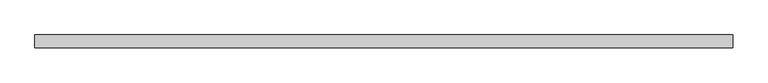
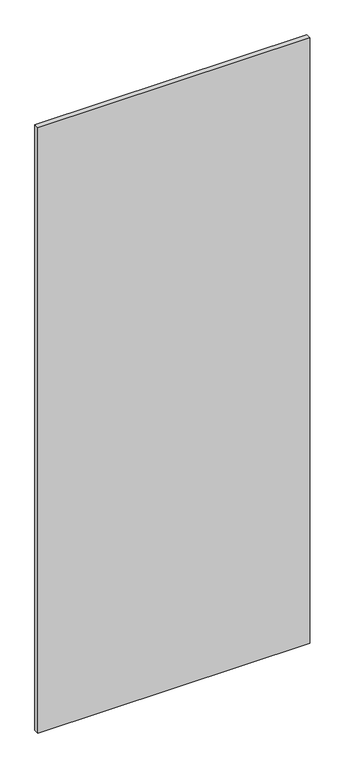
"""IFC4 building model written with IfcOpenShell, lengths in millimetres: plate geometry, 系统嵌板 : 玻璃."""

from ifc_helpers import new_model, si_unit, origin, origin_with_axes, place, context, project, spatial, polyline, outline, extrude, source, transform, mapped, element, save


def plate_81ff145c(model_context):
    return source(origin(), model_context, "Body", "SweptSolid", [
        extrude(outline(polyline([(680.0, -12.5), (-680.0, -12.5), (-680.0, 12.5), (680.0, 12.5), (680.0, -12.5)])), origin_with_axes(), (0.0, 0.0, 1.0), 3200.0),
    ])


if __name__ == "__main__":
    model = new_model("IFC4")
    model_context = context("Model", 3, world=origin())
    ifc_project = project(units=[si_unit("LENGTHUNIT", "METRE", prefix="MILLI")], contexts=[model_context])
    site = spatial("IfcSite", under=ifc_project)
    building = spatial("IfcBuilding", under=site)
    placement = place(None, origin())
    plate_shape = plate_81ff145c(model_context)
    element("IfcPlate", 1, ObjectType="系统嵌板 : 玻璃", at=placement, inside=building, context=model_context, shape_type="MappedRepresentation", body=[
        mapped(plate_shape, transform((0.0, 0.0, 0.0), x_axis=(1.0, 0.0, 0.0), y_axis=(0.0, 1.0, 0.0), z_axis=(0.0, 0.0, 1.0))),
    ])
    save(model, "model.ifc")

# Revit data of these elements
# Type "系统嵌板 : 玻璃"
#   Construction Type Id = "GSP4R"
#   Analytic Construction = "1/8 英寸 Pilkington 单层玻璃"
#   Visual Light Transmittance = 0.9
#   Solar Heat Gain Coefficient = 0.86
#   Heat Transfer Coefficient (U) = 6.7069 W/(m²·K)
# Element 1 (IfcPlate, "系统嵌板 : 玻璃")
#   Materials on its faces: "玻璃"
# Materials
#   "玻璃": class "玻璃", colour RGB 0 128 192, transparency 0.9, Description = "钠钙玻璃", Cost = 0
